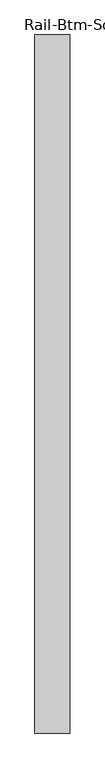
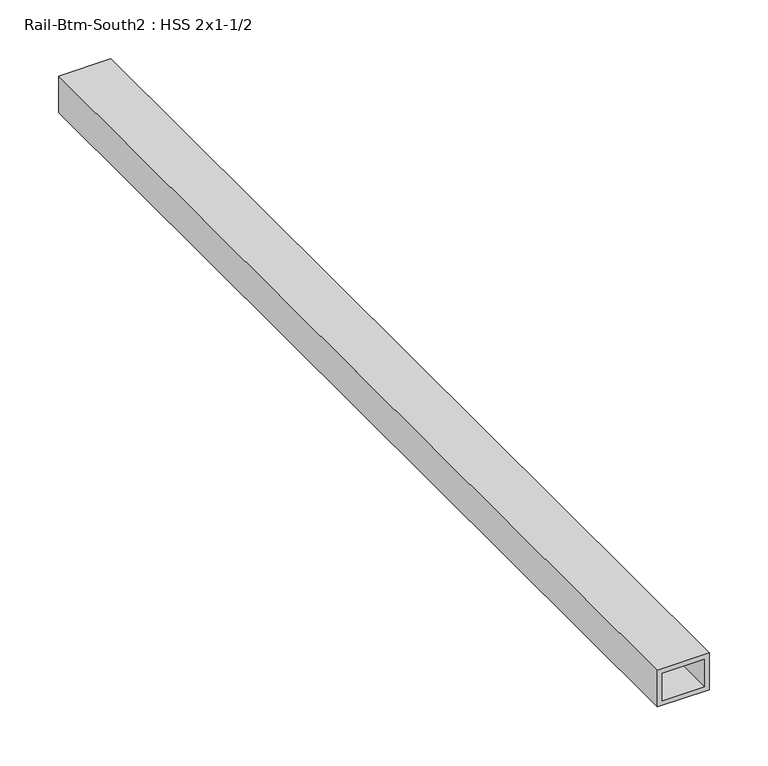
"""IFC4 building model written with IfcOpenShell, lengths in millimetres: proxy geometry, Rail-Btm-South2 : HSS 2x1-1/2."""

from ifc_helpers import new_model, si_unit, frame, origin, place, context, project, spatial, polyline, outline, extrude, source, transform, mapped, element, save


def rail_btm_south2_hss_2x1_1_2_3b7ee801(model_context):
    return source(origin(), model_context, "Body", "SweptSolid", [
        extrude(outline(polyline([(50.8, 587416.6934739), (88.9, 587416.6934739), (88.9, 587365.8934739), (50.8, 587365.8934739), (50.8, 587416.6934739)]), holes=[polyline([(84.1375, 587411.9309739), (55.5625, 587411.9309739), (55.5625, 587370.6559739), (84.1375, 587370.6559739), (84.1375, 587411.9309739)])]), frame((0.0, -533937.9163841, 0.0), z_axis=(0.0, 1.0, 0.0), x_axis=(0.0, 0.0, 1.0)), (0.0, 0.0, 1.0), 1016.0),
    ])


if __name__ == "__main__":
    model = new_model("IFC4")
    model_context = context("Model", 3, world=origin())
    ifc_project = project(units=[si_unit("LENGTHUNIT", "METRE", prefix="MILLI")], contexts=[model_context])
    site = spatial("IfcSite", under=ifc_project)
    building = spatial("IfcBuilding", under=site)
    placement = place(None, origin())
    rail_btm_south2_hss_2x1_1_2_shape = rail_btm_south2_hss_2x1_1_2_3b7ee801(model_context)
    element("IfcBuildingElementProxy", 1, Name="Rail-Btm-South2 : HSS 2x1-1/2", ObjectType="Rail-Btm-South2 : HSS 2x1-1/2", at=placement, inside=building, context=model_context, shape_type="MappedRepresentation", body=[
        mapped(rail_btm_south2_hss_2x1_1_2_shape, transform((0.0, 0.0, 0.0), x_axis=(1.0, 0.0, 0.0), y_axis=(0.0, 1.0, 0.0), z_axis=(0.0, 0.0, 1.0))),
    ])
    save(model, "model.ifc")

# Revit data of these elements
# Element 1 (IfcBuildingElementProxy, "Rail-Btm-South2 : HSS 2x1-1/2")
#   Materials on its faces: "1-1/2\"X2\" GALV. STL HSS TUBING"
# Materials
#   "1-1/2\"X2\" GALV. STL HSS TUBING": class "Generic", colour RGB 211 211 207, transparency 0, Cost = 0
